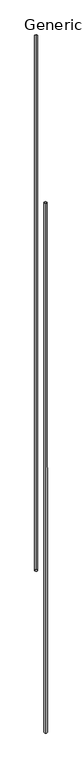
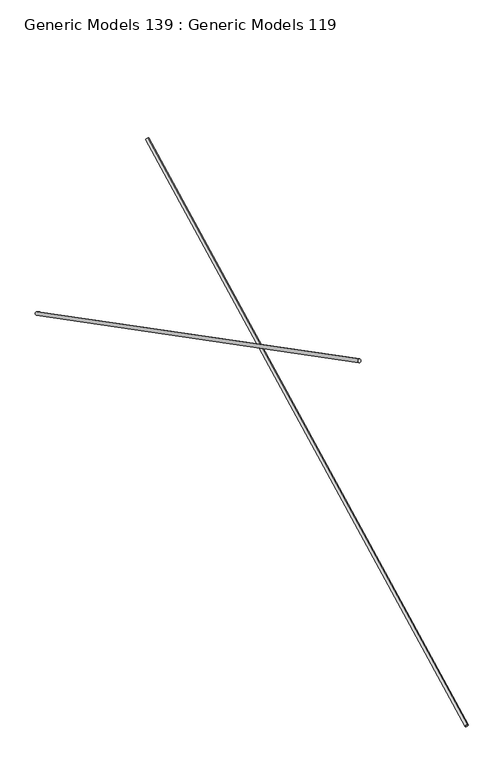
"""IFC4 building model written with IfcOpenShell, lengths in millimetres: proxy geometry, Generic Models 139 : Generic Models 119."""

import ifcopenshell
import ifcopenshell.guid

model = None  # the IFC model being written
_history = None  # IfcOwnerHistory: only IFC2X3 demands one
_inside = {}  # id of a spatial element -> (the spatial element, [elements in it])
_under = {}  # id of a project, library or spatial element -> (it, [spatial elements below it])
_declared = {}  # id of a project -> (the project, [libraries it declares])
_typed = {}  # id of a type object -> (the type object, [elements of that type])
_made_of = {}  # id of a material, layer set ... -> (it, [elements and type objects made of it])


def new_model(schema):
    """Start an empty IFC model of exactly this schema.

    Asked for "IFC4X3", IfcOpenShell would pick the latest addendum, in which some entities
    have other attributes; the version numbers below select the first issue.
    IFC2X3 requires an IfcOwnerHistory on every rooted entity: one is made here for all.
    """
    global model, _history
    if schema == "IFC4X3":
        model = ifcopenshell.file(schema_version=(4, 3, 0, 0))
    else:
        model = ifcopenshell.file(schema=schema)
    _inside.clear()
    _under.clear()
    _declared.clear()
    _typed.clear()
    _made_of.clear()
    _history = None
    if model.schema == "IFC2X3":
        org = make("IfcOrganization", Name="unknown")
        user = make(
            "IfcPersonAndOrganization",
            ThePerson=make("IfcPerson", FamilyName="unknown"),
            TheOrganization=org,
        )
        app = make(
            "IfcApplication",
            ApplicationDeveloper=org,
            Version="unknown",
            ApplicationFullName="unknown",
            ApplicationIdentifier="unknown",
        )
        _history = make(
            "IfcOwnerHistory",
            OwningUser=user,
            OwningApplication=app,
            ChangeAction="ADDED",
            CreationDate=0,
        )
    return model


def make(cls, **values):
    """One entity of the class cls with the attributes given. An attribute that is None is left unset."""
    return model.create_entity(
        cls, **{name: value for name, value in values.items() if value is not None}
    )


def rooted(cls, **values):
    """An entity with a GlobalId (a new one), such as an element, a storey or a relation."""
    return make(cls, GlobalId=ifcopenshell.guid.new(), OwnerHistory=_history, **values)


def si_unit(unit_type, name, prefix=None):
    """IfcSIUnit, for example si_unit("LENGTHUNIT", "METRE", prefix="MILLI")."""
    return make("IfcSIUnit", UnitType=unit_type, Prefix=prefix, Name=name)


def assignment(units):
    """IfcUnitAssignment: the units of a project."""
    return None if units is None else make("IfcUnitAssignment", Units=units)


def point(xyz):
    """IfcCartesianPoint."""
    return None if xyz is None else make("IfcCartesianPoint", Coordinates=xyz)


def direction(xyz):
    """IfcDirection."""
    return None if xyz is None else make("IfcDirection", DirectionRatios=xyz)


def frame(location, z_axis=None, x_axis=None):
    """IfcAxis2Placement3D, a coordinate frame: its origin and axes. An axis left out is left unset."""
    return make(
        "IfcAxis2Placement3D",
        Location=point(location),
        Axis=direction(z_axis),
        RefDirection=direction(x_axis),
    )


def origin():
    """The frame at (0, 0, 0) with its axes left unset."""
    return frame((0.0, 0.0, 0.0))


def place(relative_to, where):
    """IfcLocalPlacement: puts the frame where relative to a parent placement (None: the world)."""
    return make(
        "IfcLocalPlacement", PlacementRelTo=relative_to, RelativePlacement=where
    )


def context(
    kind, dimensions, precision=None, world=None, true_north=None, identifier=None
):
    """IfcGeometricRepresentationContext, for example the 3D "Model" context."""
    return make(
        "IfcGeometricRepresentationContext",
        ContextIdentifier=identifier,
        ContextType=kind,
        CoordinateSpaceDimension=dimensions,
        Precision=precision,
        WorldCoordinateSystem=world,
        TrueNorth=true_north,
    )


def project(units=None, contexts=None):
    """IfcProject with its units and contexts."""
    return rooted(
        "IfcProject",
        Name="project",
        RepresentationContexts=contexts,
        UnitsInContext=assignment(units),
    )


def spatial(cls, under=None, at=None, **own):
    """A site, building, storey or space (cls), placed at a placement, below another one or the project."""
    s = rooted(cls, ObjectPlacement=at, **own)
    if under is not None:
        _under.setdefault(under.id(), (under, []))[1].append(s)
    return s


def circle_curve(where, radius):
    """IfcCircle in the frame where."""
    return make("IfcCircle", Position=where, Radius=radius)


def trimmed(basis, trim1, trim2, sense, master):
    """IfcTrimmedCurve: the piece of a basis curve between two trims."""
    return make(
        "IfcTrimmedCurve",
        BasisCurve=basis,
        Trim1=trim1,
        Trim2=trim2,
        SenseAgreement=sense,
        MasterRepresentation=master,
    )


def shape(context_of_items, identifier, shape_type, items):
    """IfcShapeRepresentation: the items that make up one representation, for example the "Body"."""
    return make(
        "IfcShapeRepresentation",
        ContextOfItems=context_of_items,
        RepresentationIdentifier=identifier,
        RepresentationType=shape_type,
        Items=items,
    )


def source(mapping_origin, context_of_items, identifier, shape_type, items):
    """IfcRepresentationMap: a shape defined once, which mapped items show again and again."""
    return make(
        "IfcRepresentationMap",
        MappingOrigin=mapping_origin,
        MappedRepresentation=shape(context_of_items, identifier, shape_type, items),
    )


def transform(
    local_origin,
    x_axis=None,
    y_axis=None,
    z_axis=None,
    scale=None,
    scale2=None,
    scale3=None,
    uniform=True,
):
    """IfcCartesianTransformationOperator3D, or its non-uniform kind. x_axis, y_axis, z_axis: its Axis1, 2, 3."""
    if uniform:
        return make(
            "IfcCartesianTransformationOperator3D",
            Axis1=direction(x_axis),
            Axis2=direction(y_axis),
            LocalOrigin=point(local_origin),
            Scale=scale,
            Axis3=direction(z_axis),
        )
    return make(
        "IfcCartesianTransformationOperator3DnonUniform",
        Axis1=direction(x_axis),
        Axis2=direction(y_axis),
        LocalOrigin=point(local_origin),
        Scale=scale,
        Axis3=direction(z_axis),
        Scale2=scale2,
        Scale3=scale3,
    )


def mapped(mapping_source, mapping_target):
    """IfcMappedItem: shows the shape of a source again, moved by a transform."""
    return make(
        "IfcMappedItem", MappingSource=mapping_source, MappingTarget=mapping_target
    )


def made_of(thing, what):
    """Note that an element or type object is made of a material, layer set ...; save() writes the relation."""
    if what is not None:
        _made_of.setdefault(what.id(), (what, []))[1].append(thing)
    return thing


def element(
    cls,
    number,
    at=None,
    inside=None,
    cuts=None,
    type_object=None,
    material=None,
    context=None,
    identifier="Body",
    shape_type=None,
    held_by="IfcProductDefinitionShape",
    body=None,
    shapes=None,
    **own,
):
    """One element of the class cls, such as IfcWall. Its Tag is "e" and its number.

    at: its placement. inside: the storey or other place that contains it. cuts: it is an
    opening in that element (IfcRelVoidsElement). A single representation is given by context,
    identifier, shape_type and body (its items); several are given by shapes. held_by: the class
    of the entity that holds the representations. save() writes the other relations.
    """
    e = rooted(cls, Tag="e%d" % number, ObjectPlacement=at, **own)
    if body is not None:
        shapes = [shape(context, identifier, shape_type, body)]
    if shapes is not None:
        e.Representation = make(held_by, Representations=shapes)
    if inside is not None:
        _inside.setdefault(inside.id(), (inside, []))[1].append(e)
    if cuts is not None:
        rooted(
            "IfcRelVoidsElement", RelatingBuildingElement=cuts, RelatedOpeningElement=e
        )
    if type_object is not None:
        _typed.setdefault(type_object.id(), (type_object, []))[1].append(e)
    return made_of(e, material)


def aggregate(whole, parts):
    """IfcRelAggregates: a whole, such as a stair, and the parts it consists of."""
    return rooted("IfcRelAggregates", RelatingObject=whole, RelatedObjects=parts)


def save(model, path):
    """Write the relations noted so far, then the file.

    IfcRelAggregates (storeys below a building ...), IfcRelContainedInSpatialStructure (elements
    in a storey), IfcRelDefinesByType, IfcRelAssociatesMaterial and IfcRelDeclares: one each for
    every whole, place, type object, material and project.
    """
    for whole, parts in _under.values():
        aggregate(whole, parts)
    for where, things in _inside.values():
        rooted(
            "IfcRelContainedInSpatialStructure",
            RelatedElements=things,
            RelatingStructure=where,
        )
    for kind, things in _typed.values():
        rooted("IfcRelDefinesByType", RelatedObjects=things, RelatingType=kind)
    for what, things in _made_of.values():
        rooted("IfcRelAssociatesMaterial", RelatedObjects=things, RelatingMaterial=what)
    for by, libraries in _declared.values():
        rooted("IfcRelDeclares", RelatingContext=by, RelatedDefinitions=libraries)
    model.write(path)


def plane_surface(at):
    """IfcPlane: the flat surface through the origin of the frame at, square to its z axis."""
    return make("IfcPlane", Position=at)


def extruded_surface(curve, direction_of_extrusion, depth):
    """IfcSurfaceOfLinearExtrusion: the curve pushed along a direction by depth."""
    return make(
        "IfcSurfaceOfLinearExtrusion",
        SweptCurve=make("IfcArbitraryOpenProfileDef", ProfileType="CURVE", Curve=curve),
        ExtrudedDirection=direction(direction_of_extrusion),
        Depth=depth,
    )


def advanced_brep(points, edges, surfaces, faces):
    """IfcAdvancedBrep: a solid bounded by faces that lie on surfaces and meet in shared edges.

    An edge is (start, end): straight between two places in points (the first is 0);
    or (start, end, curve); or (start, end, curve, False) where it runs against its curve.
    A face is (place in surfaces, loops), or (place, loops, False) where it looks against
    its surface's normal. A loop lists edges by number (the first is 1), with a minus sign
    where the edge is run from its end to its start. The first loop is the outer one.
    """
    corners = [point(p) for p in points]
    vertices = [make("IfcVertexPoint", VertexGeometry=c) for c in corners]
    made = []
    for start, end, *more in edges:
        made.append(
            make(
                "IfcEdgeCurve",
                EdgeStart=vertices[start],
                EdgeEnd=vertices[end],
                EdgeGeometry=more[0] if more else make("IfcPolyline", Points=[corners[start], corners[end]]),
                SameSense=more[1] if len(more) > 1 else True,
            )
        )
    hull = []
    for where, loops, *sense in faces:
        bounds = []
        for j, loop in enumerate(loops):
            ring = [make("IfcOrientedEdge", EdgeElement=made[abs(k) - 1], Orientation=k > 0) for k in loop]
            bounds.append(
                make(
                    "IfcFaceOuterBound" if j == 0 else "IfcFaceBound",
                    Bound=make("IfcEdgeLoop", EdgeList=ring),
                    Orientation=True,
                )
            )
        hull.append(make("IfcAdvancedFace", Bounds=bounds, FaceSurface=surfaces[where], SameSense=sense[0] if sense else True))
    return make("IfcAdvancedBrep", Outer=make("IfcClosedShell", CfsFaces=hull))


def generic_models_139_generic_models_119_bb35afc2(model_context):
    return source(origin(), model_context, "Body", "AdvancedBrep", [
        advanced_brep(
        [(32003.9965778, 30877.5659964, 266463.8403309), (32003.9965778, 30886.2933954, 266446.9070794), (32002.4450787, 34140.039121, 268145.3192042), (32002.4450787, 34148.76652, 268128.3859527)],
        [
            (0, 1, circle_curve(frame((32003.9965778, 30881.9296959, 266455.3737052), z_axis=(0.0, -0.8888845937971532, -0.4581311808969894), x_axis=(0.0, 0.4581311808969894, -0.8888845937971532)), 9.525)),
            (1, 0, circle_curve(frame((32003.9965778, 30881.9296959, 266455.3737052), z_axis=(0.0, -0.8888845937971532, -0.4581311808969894), x_axis=(0.0, 0.4581311808969894, -0.8888845937971532)), 9.525)),
            (2, 3, circle_curve(frame((32002.4450787, 34144.4028205, 268136.8525784), z_axis=(0.0, 0.8888845937971532, 0.4581311808969894), x_axis=(0.0, 0.4581311808969894, -0.8888845937971532)), 9.525)),
            (3, 2, circle_curve(frame((32002.4450787, 34144.4028205, 268136.8525784), z_axis=(0.0, 0.8888845937971532, 0.4581311808969894), x_axis=(0.0, 0.4581311808969894, -0.8888845937971532)), 9.525)),
            (3, 1),
            (0, 2),
        ],
        [
            plane_surface(frame((32003.9965778, 30881.9296959, 266455.3737052), z_axis=(0.0, -0.8888845937971532, -0.4581311808969894), x_axis=(-1.0, 0.0, 0.0))),
            plane_surface(frame((32002.4450787, 34144.4028205, 268136.8525784), z_axis=(0.0, 0.8888845937971532, 0.4581311808969894), x_axis=(-1.0, 0.0, 0.0))),
            extruded_surface(trimmed(circle_curve(frame((32002.4450787, 34144.4028205, 268136.8525784), z_axis=(0.0, -0.8888845937971532, -0.4581311808969894), x_axis=(0.0, 0.4581311808969894, -0.8888845937971532)), 9.525), [point((32002.4450787, 34140.039121, 268145.3192042))], [point((32002.4450787, 34148.76652, 268128.3859527))], True, "CARTESIAN"), (1.55149910000182, -3262.473124600001, -1681.478873200016), 3670.3003278893602),
            extruded_surface(trimmed(circle_curve(frame((32002.4450787, 34144.4028205, 268136.8525784), z_axis=(0.0, -0.8888845937971532, -0.4581311808969894), x_axis=(0.0, 0.4581311808969894, -0.8888845937971532)), 9.525), [point((32002.4450787, 34148.76652, 268128.3859527))], [point((32002.4450787, 34140.039121, 268145.3192042))], True, "CARTESIAN"), (1.55149910000182, -3262.473124600001, -1681.478873200016), 3670.3003278893602),
        ],
        [
            (0, [[1, 2]]),
            (1, [[3, 4]]),
            (2, [[-4, 5, -1, 6]]),
            (3, [[-3, -6, -2, -5]]),
        ],
    ),
        advanced_brep(
        [(31945.3483901, 35168.4634288, 266435.1980333), (31945.3483901, 35177.2143812, 266452.1191247), (31945.2937775, 31874.4909796, 268138.7167634), (31945.2937775, 31883.241932, 268155.6378548)],
        [
            (0, 1, circle_curve(frame((31945.3483901, 35172.838905, 266443.658579), z_axis=(0.0, 0.8882462650221944, -0.459367579041144), x_axis=(0.0, 0.459367579041144, 0.8882462650221944)), 9.525)),
            (1, 0, circle_curve(frame((31945.3483901, 35172.838905, 266443.658579), z_axis=(0.0, 0.8882462650221944, -0.459367579041144), x_axis=(0.0, 0.459367579041144, 0.8882462650221944)), 9.525)),
            (2, 3, circle_curve(frame((31945.2937775, 31878.8664558, 268147.1773091), z_axis=(0.0, -0.8882462650221944, 0.459367579041144), x_axis=(0.0, 0.459367579041144, 0.8882462650221944)), 9.525)),
            (3, 2, circle_curve(frame((31945.2937775, 31878.8664558, 268147.1773091), z_axis=(0.0, -0.8882462650221944, 0.459367579041144), x_axis=(0.0, 0.459367579041144, 0.8882462650221944)), 9.525)),
            (3, 1),
            (0, 2),
        ],
        [
            plane_surface(frame((31945.3483901, 35172.838905, 266443.658579), z_axis=(0.0, 0.8882462650221944, -0.459367579041144), x_axis=(-1.0, 0.0, 0.0))),
            plane_surface(frame((31945.2937775, 31878.8664558, 268147.1773091), z_axis=(0.0, -0.8882462650221944, 0.459367579041144), x_axis=(-1.0, 0.0, 0.0))),
            extruded_surface(trimmed(circle_curve(frame((31945.2937775, 31878.8664558, 268147.1773091), z_axis=(0.0, 0.8882462650221944, -0.459367579041144), x_axis=(0.0, 0.459367579041144, 0.8882462650221944)), 9.525), [point((31945.2937775, 31874.4909796, 268138.7167634))], [point((31945.2937775, 31883.241932, 268155.6378548))], True, "CARTESIAN"), (0.05461260000083712, 3293.9724491999987, -1703.5187301000115), 3708.400000387327),
            extruded_surface(trimmed(circle_curve(frame((31945.2937775, 31878.8664558, 268147.1773091), z_axis=(0.0, 0.8882462650221944, -0.459367579041144), x_axis=(0.0, 0.459367579041144, 0.8882462650221944)), 9.525), [point((31945.2937775, 31883.241932, 268155.6378548))], [point((31945.2937775, 31874.4909796, 268138.7167634))], True, "CARTESIAN"), (0.05461260000083712, 3293.9724491999987, -1703.5187301000115), 3708.400000387327),
        ],
        [
            (0, [[1, 2]]),
            (1, [[3, 4]]),
            (2, [[-4, 5, -1, 6]]),
            (3, [[-3, -6, -2, -5]]),
        ],
    ),
    ])


if __name__ == "__main__":
    model = new_model("IFC4")
    model_context = context("Model", 3, world=origin())
    ifc_project = project(units=[si_unit("LENGTHUNIT", "METRE", prefix="MILLI")], contexts=[model_context])
    site = spatial("IfcSite", under=ifc_project)
    building = spatial("IfcBuilding", under=site)
    placement = place(None, origin())
    generic_models_139_generic_models_119_shape = generic_models_139_generic_models_119_bb35afc2(model_context)
    element("IfcBuildingElementProxy", 1, Name="Generic Models 139 : Generic Models 119", ObjectType="Generic Models 139 : Generic Models 119", at=placement, inside=building, context=model_context, shape_type="MappedRepresentation", body=[
        mapped(generic_models_139_generic_models_119_shape, transform((0.0, 0.0, 0.0), x_axis=(1.0, 0.0, 0.0), y_axis=(0.0, 1.0, 0.0), z_axis=(0.0, 0.0, 1.0))),
    ])
    save(model, "model.ifc")

# Revit data of these elements
# Element 1 (IfcBuildingElementProxy, "Generic Models 139 : Generic Models 119")
#   Materials on its faces: "3/4\" DIA. ROD"
# Materials
#   "3/4\" DIA. ROD": class "Metal", colour RGB 199 199 199, transparency 0, Description = "Carbon steel", Cost = 0
